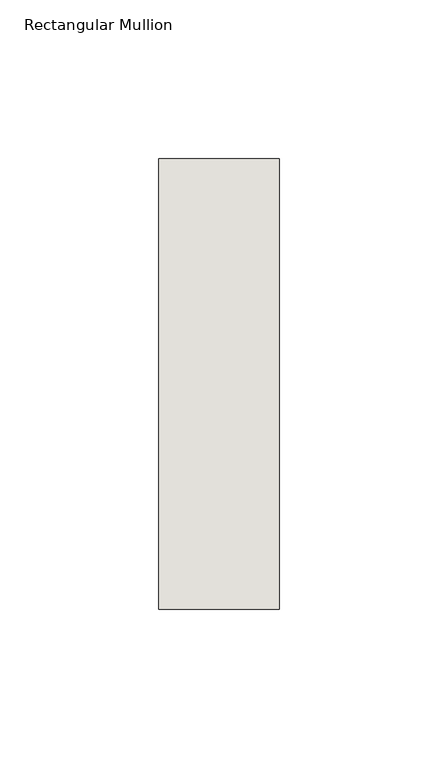
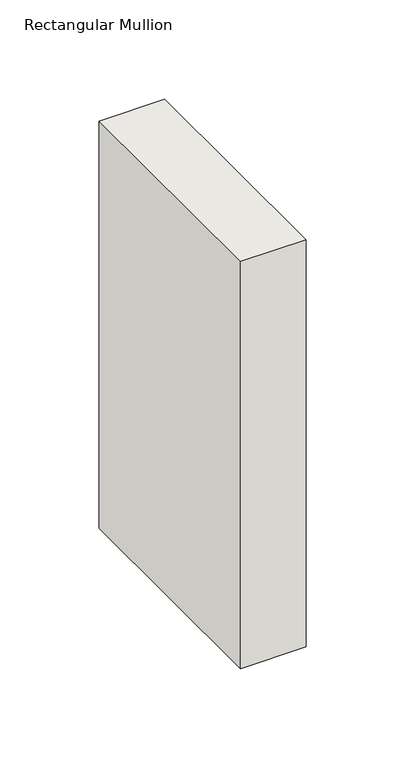
"""IFC4 building model written with IfcOpenShell, lengths in millimetres: wall geometry, Rectangular Mullion : NLRS_21_CWM_hsb-regel 38x142_gen_rsf."""

from ifc_helpers import new_model, si_unit, frame, origin, place, context, project, spatial, polyline, outline, extrude, source, transform, mapped, element, save


def rectangular_mullion_56763ec6(model_context):
    return source(origin(), model_context, "Body", "SweptSolid", [
        extrude(outline(polyline([(-38.0, -71.0), (-38.0, 71.0), (0.0, 71.0), (0.0, -71.0), (-38.0, -71.0)])), frame((0.0, 0.0, -250.0000003), z_axis=(0.0, 0.0, 1.0), x_axis=(1.0, 0.0, 0.0)), (0.0, 0.0, 1.0), 250.0000003),
    ])


if __name__ == "__main__":
    model = new_model("IFC4")
    model_context = context("Model", 3, world=origin())
    ifc_project = project(units=[si_unit("LENGTHUNIT", "METRE", prefix="MILLI")], contexts=[model_context])
    site = spatial("IfcSite", under=ifc_project)
    building = spatial("IfcBuilding", under=site)
    placement = place(None, origin())
    rectangular_mullion_shape = rectangular_mullion_56763ec6(model_context)
    element("IfcWall", 1, ObjectType="Rectangular Mullion : NLRS_21_CWM_hsb-regel 38x142_gen_rsf", at=placement, inside=building, context=model_context, shape_type="MappedRepresentation", body=[
        mapped(rectangular_mullion_shape, transform((0.0, 0.0, 0.0), x_axis=(1.0, 0.0, 0.0), y_axis=(0.0, 1.0, 0.0), z_axis=(0.0, 0.0, 1.0))),
    ])
    save(model, "model.ifc")

# Revit data of these elements
# Type "Rectangular Mullion : NLRS_21_CWM_hsb-regel 38x142_gen_rsf"
#   Type IfcGUID = "07M7mRoiH1CR8m_RSKIwpF"
#   Assembly Code = "21.10"
#   IfcExportAs = "IfcWall"
#   built-in parameter 1007322 = 0.465879 (stored number, unit not read)
#   built-in parameter 1007321 = 0.062336 (stored number, unit not read)
#   built-in parameter 1007320 = 0.062336 (stored number, unit not read)
# Element 1 (IfcWall, "Rectangular Mullion : NLRS_21_CWM_hsb-regel 38x142_gen_rsf")
#   Materials on its faces: "NLRS_i2_hout naaldhout vuren_gen_rsf"
# Materials
#   "NLRS_i2_hout naaldhout vuren_gen_rsf": class "I - Hout", colour RGB 234 199 147, transparency 0, Keynote = "i2", Manufacturer = "Revit Standards Foundation", URL = "www.revitstandards.org", Description = "hout vuren", Cost = 0
